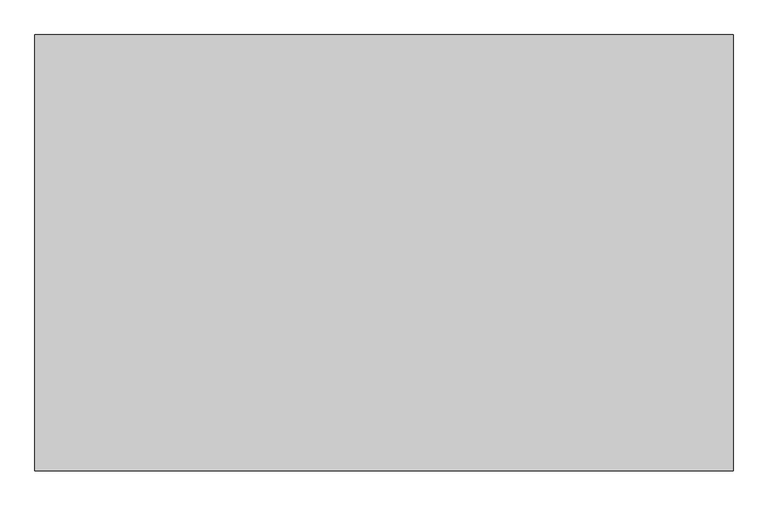
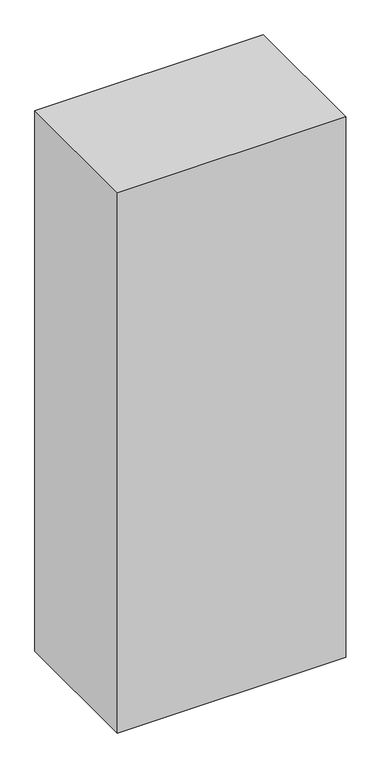
"""IFC4 building model written with IfcOpenShell, lengths in millimetres: proxy geometry, Space Planning Box_hec : Space Planning Box_hec."""

from ifc_helpers import new_model, si_unit, origin, origin_with_axes, place, context, project, spatial, polyline, outline, extrude, source, transform, mapped, element, save


def generic_models_7a053eeb(model_context):
    return source(origin(), model_context, "Body", "SweptSolid", [
        extrude(outline(polyline([(1200.0, 750.0), (1200.0, -750.0), (-1200.0, -750.0), (-1200.0, 750.0), (1200.0, 750.0)])), origin_with_axes(), (0.0, 0.0, 1.0), 6000.0),
    ])


if __name__ == "__main__":
    model = new_model("IFC4")
    model_context = context("Model", 3, world=origin())
    ifc_project = project(units=[si_unit("LENGTHUNIT", "METRE", prefix="MILLI")], contexts=[model_context])
    site = spatial("IfcSite", under=ifc_project)
    building = spatial("IfcBuilding", under=site)
    placement = place(None, origin())
    generic_models_shape = generic_models_7a053eeb(model_context)
    element("IfcBuildingElementProxy", 1, Name="Space Planning Box_hec : Space Planning Box_hec", ObjectType="Space Planning Box_hec : Space Planning Box_hec", at=placement, inside=building, context=model_context, shape_type="MappedRepresentation", body=[
        mapped(generic_models_shape, transform((0.0, 0.0, 0.0), x_axis=(1.0, 0.0, 0.0), y_axis=(0.0, 1.0, 0.0), z_axis=(0.0, 0.0, 1.0))),
    ])
    save(model, "model.ifc")

# Revit data of these elements
# Type "Space Planning Box_hec : Space Planning Box_hec"
#   Type Comments = "..."
#   Room Name [instance default] = "?"
#   Interior Finish [instance default] = ""
#   Exterior Finish [instance default] = ""
#   Department [instance default] = ""
#   Assembly Code = "..."
#   Width [instance default] = 1524 mm
#   Program Area [instance default] = 0 m²
#   Length [instance default] = 1524 mm
#   Height [instance default] = 1524 mm
#   Area [instance default] = 2.32258 m²
#   Fill Color [instance default] = Cyan
#   Default Elevation = 0
# Element 1 (IfcBuildingElementProxy, "Space Planning Box_hec : Space Planning Box_hec")
#   Room Name = "Shower Room (F)"
#   Interior Finish = "IF5"
#   Exterior Finish = "EF1"
#   Department = "AR"
#   Width = 2400 mm
#   Program Area = 31.5 m²
#   Length = 1500 mm
#   Height = 6000 mm
#   Area = 3.6 m²
#   Fill Color = Lavender
#   Materials on its faces: "Lavender"
# Materials
#   "Cyan": class "Generic", colour RGB 0 255 255, transparency 0.2, Cost = 0
#   "Lavender": class "Generic", colour RGB 186 85 211, transparency 0.2, Cost = 0
